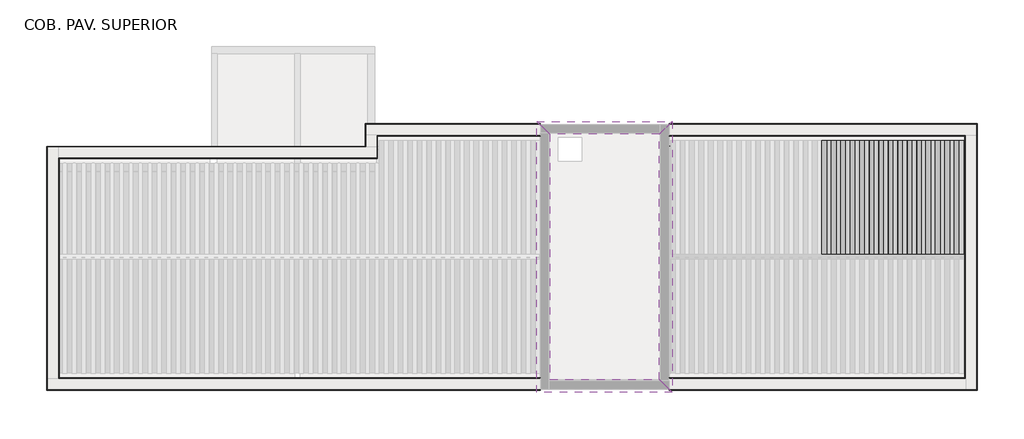
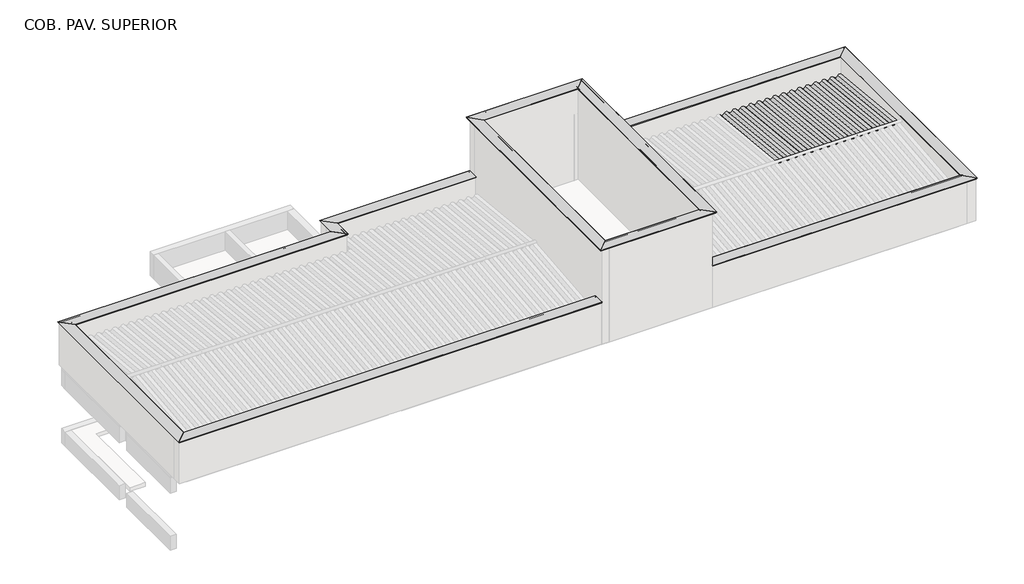
# One storey, part 7 of 7: 25 beams, 9 columns, 4 proxies.
"""IFC4 building model written with IfcOpenShell, lengths in millimetres."""

import ifcopenshell
import ifcopenshell.guid

model = None  # the IFC model being written
_history = None  # IfcOwnerHistory: only IFC2X3 demands one
_inside = {}  # id of a spatial element -> (the spatial element, [elements in it])
_under = {}  # id of a project, library or spatial element -> (it, [spatial elements below it])
_declared = {}  # id of a project -> (the project, [libraries it declares])
_typed = {}  # id of a type object -> (the type object, [elements of that type])
_made_of = {}  # id of a material, layer set ... -> (it, [elements and type objects made of it])


def new_model(schema):
    """Start an empty IFC model of exactly this schema.

    Asked for "IFC4X3", IfcOpenShell would pick the latest addendum, in which some entities
    have other attributes; the version numbers below select the first issue.
    IFC2X3 requires an IfcOwnerHistory on every rooted entity: one is made here for all.
    """
    global model, _history
    if schema == "IFC4X3":
        model = ifcopenshell.file(schema_version=(4, 3, 0, 0))
    else:
        model = ifcopenshell.file(schema=schema)
    _inside.clear()
    _under.clear()
    _declared.clear()
    _typed.clear()
    _made_of.clear()
    _history = None
    if model.schema == "IFC2X3":
        org = make("IfcOrganization", Name="unknown")
        user = make(
            "IfcPersonAndOrganization",
            ThePerson=make("IfcPerson", FamilyName="unknown"),
            TheOrganization=org,
        )
        app = make(
            "IfcApplication",
            ApplicationDeveloper=org,
            Version="unknown",
            ApplicationFullName="unknown",
            ApplicationIdentifier="unknown",
        )
        _history = make(
            "IfcOwnerHistory",
            OwningUser=user,
            OwningApplication=app,
            ChangeAction="ADDED",
            CreationDate=0,
        )
    return model


def make(cls, **values):
    """One entity of the class cls with the attributes given. An attribute that is None is left unset."""
    return model.create_entity(
        cls, **{name: value for name, value in values.items() if value is not None}
    )


def rooted(cls, **values):
    """An entity with a GlobalId (a new one), such as an element, a storey or a relation."""
    return make(cls, GlobalId=ifcopenshell.guid.new(), OwnerHistory=_history, **values)


def si_unit(unit_type, name, prefix=None):
    """IfcSIUnit, for example si_unit("LENGTHUNIT", "METRE", prefix="MILLI")."""
    return make("IfcSIUnit", UnitType=unit_type, Prefix=prefix, Name=name)


def assignment(units):
    """IfcUnitAssignment: the units of a project."""
    return None if units is None else make("IfcUnitAssignment", Units=units)


def point(xyz):
    """IfcCartesianPoint."""
    return None if xyz is None else make("IfcCartesianPoint", Coordinates=xyz)


def direction(xyz):
    """IfcDirection."""
    return None if xyz is None else make("IfcDirection", DirectionRatios=xyz)


def frame(location, z_axis=None, x_axis=None):
    """IfcAxis2Placement3D, a coordinate frame: its origin and axes. An axis left out is left unset."""
    return make(
        "IfcAxis2Placement3D",
        Location=point(location),
        Axis=direction(z_axis),
        RefDirection=direction(x_axis),
    )


def frame_2d(location, x_axis=None):
    """IfcAxis2Placement2D, a coordinate frame in the plane: its origin and x axis."""
    return make(
        "IfcAxis2Placement2D", Location=point(location), RefDirection=direction(x_axis)
    )


def origin():
    """The frame at (0, 0, 0) with its axes left unset."""
    return frame((0.0, 0.0, 0.0))


def place(relative_to, where):
    """IfcLocalPlacement: puts the frame where relative to a parent placement (None: the world)."""
    return make(
        "IfcLocalPlacement", PlacementRelTo=relative_to, RelativePlacement=where
    )


def context(
    kind, dimensions, precision=None, world=None, true_north=None, identifier=None
):
    """IfcGeometricRepresentationContext, for example the 3D "Model" context."""
    return make(
        "IfcGeometricRepresentationContext",
        ContextIdentifier=identifier,
        ContextType=kind,
        CoordinateSpaceDimension=dimensions,
        Precision=precision,
        WorldCoordinateSystem=world,
        TrueNorth=true_north,
    )


def project(units=None, contexts=None):
    """IfcProject with its units and contexts."""
    return rooted(
        "IfcProject",
        Name="project",
        RepresentationContexts=contexts,
        UnitsInContext=assignment(units),
    )


def spatial(cls, under=None, at=None, **own):
    """A site, building, storey or space (cls), placed at a placement, below another one or the project."""
    s = rooted(cls, ObjectPlacement=at, **own)
    if under is not None:
        _under.setdefault(under.id(), (under, []))[1].append(s)
    return s


def polyline(points):
    """IfcPolyline through the points."""
    return make("IfcPolyline", Points=[point(p) for p in points])


def circle_curve(where, radius):
    """IfcCircle in the frame where."""
    return make("IfcCircle", Position=where, Radius=radius)


def trimmed(basis, trim1, trim2, sense, master):
    """IfcTrimmedCurve: the piece of a basis curve between two trims."""
    return make(
        "IfcTrimmedCurve",
        BasisCurve=basis,
        Trim1=trim1,
        Trim2=trim2,
        SenseAgreement=sense,
        MasterRepresentation=master,
    )


def segment(curve, same_sense, transition):
    """IfcCompositeCurveSegment."""
    return make(
        "IfcCompositeCurveSegment",
        Transition=transition,
        SameSense=same_sense,
        ParentCurve=curve,
    )


def composite_curve(segments, self_intersect=None):
    """IfcCompositeCurve: segments joined end to end."""
    return make("IfcCompositeCurve", Segments=segments, SelfIntersect=self_intersect)


def outline(outer, holes=None, kind="AREA"):
    """IfcArbitraryClosedProfileDef: a profile drawn as a closed curve; with holes, ...WithVoids."""
    if holes is None:
        return make("IfcArbitraryClosedProfileDef", ProfileType=kind, OuterCurve=outer)
    return make(
        "IfcArbitraryProfileDefWithVoids",
        ProfileType=kind,
        OuterCurve=outer,
        InnerCurves=holes,
    )


def extrude(swept, where, along, depth):
    """IfcExtrudedAreaSolid: the profile swept, set in the frame where, extruded along a direction by depth."""
    return make(
        "IfcExtrudedAreaSolid",
        SweptArea=swept,
        Position=where,
        ExtrudedDirection=direction(along),
        Depth=depth,
    )


def faces_of(points, faces, orient=None, outer=None):
    """IfcFace entities. A face is a list of loops; a loop is a list of indices into points, from 0.

    orient and outer hold one flag for each loop. By default every Orientation is true, the
    first loop of a face is its IfcFaceOuterBound and the others are IfcFaceBound.
    """
    made = []
    for i, loops in enumerate(faces):
        bounds = []
        for j, loop in enumerate(loops):
            is_outer = j == 0 if outer is None else outer[i][j]
            bounds.append(
                make(
                    "IfcFaceOuterBound" if is_outer else "IfcFaceBound",
                    Bound=make("IfcPolyLoop", Polygon=[points[k] for k in loop]),
                    Orientation=True if orient is None else orient[i][j],
                )
            )
        made.append(make("IfcFace", Bounds=bounds))
    return made


def faceted_brep(points, faces, orient=None, outer=None, voids=None):
    """IfcFacetedBrep: a solid bounded by flat faces; with voids (closed shells), ...WithVoids."""
    shared = [point(p) for p in points]
    hull = make("IfcClosedShell", CfsFaces=faces_of(shared, faces, orient, outer))
    if voids is None:
        return make("IfcFacetedBrep", Outer=hull)
    return make(
        "IfcFacetedBrepWithVoids",
        Outer=hull,
        Voids=[
            make(cls, CfsFaces=faces_of(shared, fs, o, b)) for cls, fs, o, b in voids
        ],
    )


def shape(context_of_items, identifier, shape_type, items):
    """IfcShapeRepresentation: the items that make up one representation, for example the "Body"."""
    return make(
        "IfcShapeRepresentation",
        ContextOfItems=context_of_items,
        RepresentationIdentifier=identifier,
        RepresentationType=shape_type,
        Items=items,
    )


def source(mapping_origin, context_of_items, identifier, shape_type, items):
    """IfcRepresentationMap: a shape defined once, which mapped items show again and again."""
    return make(
        "IfcRepresentationMap",
        MappingOrigin=mapping_origin,
        MappedRepresentation=shape(context_of_items, identifier, shape_type, items),
    )


def transform(
    local_origin,
    x_axis=None,
    y_axis=None,
    z_axis=None,
    scale=None,
    scale2=None,
    scale3=None,
    uniform=True,
):
    """IfcCartesianTransformationOperator3D, or its non-uniform kind. x_axis, y_axis, z_axis: its Axis1, 2, 3."""
    if uniform:
        return make(
            "IfcCartesianTransformationOperator3D",
            Axis1=direction(x_axis),
            Axis2=direction(y_axis),
            LocalOrigin=point(local_origin),
            Scale=scale,
            Axis3=direction(z_axis),
        )
    return make(
        "IfcCartesianTransformationOperator3DnonUniform",
        Axis1=direction(x_axis),
        Axis2=direction(y_axis),
        LocalOrigin=point(local_origin),
        Scale=scale,
        Axis3=direction(z_axis),
        Scale2=scale2,
        Scale3=scale3,
    )


def mapped(mapping_source, mapping_target):
    """IfcMappedItem: shows the shape of a source again, moved by a transform."""
    return make(
        "IfcMappedItem", MappingSource=mapping_source, MappingTarget=mapping_target
    )


def made_of(thing, what):
    """Note that an element or type object is made of a material, layer set ...; save() writes the relation."""
    if what is not None:
        _made_of.setdefault(what.id(), (what, []))[1].append(thing)
    return thing


def element(
    cls,
    number,
    at=None,
    inside=None,
    cuts=None,
    type_object=None,
    material=None,
    context=None,
    identifier="Body",
    shape_type=None,
    held_by="IfcProductDefinitionShape",
    body=None,
    shapes=None,
    **own,
):
    """One element of the class cls, such as IfcWall. Its Tag is "e" and its number.

    at: its placement. inside: the storey or other place that contains it. cuts: it is an
    opening in that element (IfcRelVoidsElement). A single representation is given by context,
    identifier, shape_type and body (its items); several are given by shapes. held_by: the class
    of the entity that holds the representations. save() writes the other relations.
    """
    e = rooted(cls, Tag="e%d" % number, ObjectPlacement=at, **own)
    if body is not None:
        shapes = [shape(context, identifier, shape_type, body)]
    if shapes is not None:
        e.Representation = make(held_by, Representations=shapes)
    if inside is not None:
        _inside.setdefault(inside.id(), (inside, []))[1].append(e)
    if cuts is not None:
        rooted(
            "IfcRelVoidsElement", RelatingBuildingElement=cuts, RelatedOpeningElement=e
        )
    if type_object is not None:
        _typed.setdefault(type_object.id(), (type_object, []))[1].append(e)
    return made_of(e, material)


def aggregate(whole, parts):
    """IfcRelAggregates: a whole, such as a stair, and the parts it consists of."""
    return rooted("IfcRelAggregates", RelatingObject=whole, RelatedObjects=parts)


def save(model, path):
    """Write the relations noted so far, then the file.

    IfcRelAggregates (storeys below a building ...), IfcRelContainedInSpatialStructure (elements
    in a storey), IfcRelDefinesByType, IfcRelAssociatesMaterial and IfcRelDeclares: one each for
    every whole, place, type object, material and project.
    """
    for whole, parts in _under.values():
        aggregate(whole, parts)
    for where, things in _inside.values():
        rooted(
            "IfcRelContainedInSpatialStructure",
            RelatedElements=things,
            RelatingStructure=where,
        )
    for kind, things in _typed.values():
        rooted("IfcRelDefinesByType", RelatedObjects=things, RelatingType=kind)
    for what, things in _made_of.values():
        rooted("IfcRelAssociatesMaterial", RelatedObjects=things, RelatingMaterial=what)
    for by, libraries in _declared.values():
        rooted("IfcRelDeclares", RelatingContext=by, RelatedDefinitions=libraries)
    model.write(path)


def column_d505325c(model_context):
    return source(origin(), model_context, "Body", "SweptSolid", [
        extrude(outline(polyline([(30.0, 80.0), (30.0, -80.0), (-30.0, -80.0), (-30.0, 80.0), (30.0, 80.0)])), frame((0.0, 0.0, 6710.0), z_axis=(0.0, 0.0, 1.0), x_axis=(1.0, 0.0, 0.0)), (0.0, 0.0, 1.0), 750.0),
    ])


def column_4db371bd(model_context):
    return source(origin(), model_context, "Body", "SweptSolid", [
        extrude(outline(polyline([(30.0, 80.0), (30.0, -80.0), (-30.0, -80.0), (-30.0, 80.0), (30.0, 80.0)])), frame((0.0, 0.0, 6710.0), z_axis=(0.0, 0.0, 1.0), x_axis=(1.0, 0.0, 0.0)), (0.0, 0.0, 1.0), 660.0),
    ])


def column_d0cf395a(model_context):
    return source(origin(), model_context, "Body", "SweptSolid", [
        extrude(outline(polyline([(30.0, 80.0), (30.0, -80.0), (-30.0, -80.0), (-30.0, 80.0), (30.0, 80.0)])), frame((0.0, 0.0, 6710.0), z_axis=(0.0, 0.0, 1.0), x_axis=(1.0, 0.0, 0.0)), (0.0, 0.0, 1.0), 520.0),
    ])


model = new_model("IFC4")

# Units and contexts
model_context = context("Model", 3, world=origin())
ifc_project = project(units=[si_unit("LENGTHUNIT", "METRE", prefix="MILLI")], contexts=[model_context])

# Site, building, storey
site = spatial("IfcSite", under=ifc_project)
building = spatial("IfcBuilding", under=site)
storey = spatial("IfcBuildingStorey", under=building, Name="COB. PAV. SUPERIOR", Elevation=6650.0)

# Beams
placement = place(None, origin())
element("IfcBeam", 1, ObjectType="Madeira de lei : Berço 6x12cm", at=placement, inside=storey, context=model_context, shape_type="SweptSolid", body=[
    extrude(outline(polyline([(9090.718693, -7711.5607799), (9090.718693, -7831.5607799), (7090.718693, -7831.5607799), (7090.718693, -7711.5607799), (9090.718693, -7711.5607799)])), frame((0.0, 0.0, 6650.0), z_axis=(0.0, 0.0, 1.0), x_axis=(1.0, 0.0, 0.0)), (0.0, 0.0, 1.0), 60.0),
])
element("IfcBeam", 2, ObjectType="Madeira de lei : Berço 6x12cm", at=placement, inside=storey, context=model_context, shape_type="SweptSolid", body=[
    extrude(outline(polyline([(10730.718693, -7711.5607799), (10730.718693, -7831.5607799), (9090.718693, -7831.5607799), (9090.718693, -7711.5607799), (10730.718693, -7711.5607799)])), frame((0.0, 0.0, 6650.0), z_axis=(0.0, 0.0, 1.0), x_axis=(1.0, 0.0, 0.0)), (0.0, 0.0, 1.0), 60.0),
])
element("IfcBeam", 3, ObjectType="Madeira de lei : Berço 6x12cm", at=placement, inside=storey, context=model_context, shape_type="SweptSolid", body=[
    extrude(outline(polyline([(9089.7186924, -6319.8711004), (9089.7186924, -6439.8711004), (7089.7186936, -6439.8711004), (7089.7186936, -6319.8711004), (9089.7186924, -6319.8711004)])), frame((0.0, 0.0, 6650.0), z_axis=(0.0, 0.0, 1.0), x_axis=(1.0, 0.0, 0.0)), (0.0, 0.0, 1.0), 60.0),
])
element("IfcBeam", 4, ObjectType="Madeira de lei : Berço 6x12cm", at=placement, inside=storey, context=model_context, shape_type="SweptSolid", body=[
    extrude(outline(polyline([(10729.718693, -6319.8711004), (10729.718693, -6439.8711004), (9089.7186936, -6439.8711004), (9089.7186936, -6319.8711004), (10729.718693, -6319.8711004)])), frame((0.0, 0.0, 6650.0), z_axis=(0.0, 0.0, 1.0), x_axis=(1.0, 0.0, 0.0)), (0.0, 0.0, 1.0), 60.0),
])
element("IfcBeam", 5, ObjectType="Madeira de lei : Berço 6x12cm", at=placement, inside=storey, context=model_context, shape_type="SweptSolid", body=[
    extrude(outline(polyline([(5089.7186924, -4899.3026908), (5089.7186924, -5019.3026908), (3089.718693, -5019.3026908), (3089.718693, -4899.3026908), (5089.7186924, -4899.3026908)])), frame((0.0, 0.0, 6650.0), z_axis=(0.0, 0.0, 1.0), x_axis=(1.0, 0.0, 0.0)), (0.0, 0.0, 1.0), 60.0),
])
element("IfcBeam", 6, ObjectType="Madeira de lei : Berço 6x12cm", at=placement, inside=storey, context=model_context, shape_type="SweptSolid", body=[
    extrude(outline(polyline([(7089.7186924, -4899.3026908), (7089.7186924, -5019.3026908), (5089.7186936, -5019.3026908), (5089.7186936, -4899.3026908), (7089.7186924, -4899.3026908)])), frame((0.0, 0.0, 6650.0), z_axis=(0.0, 0.0, 1.0), x_axis=(1.0, 0.0, 0.0)), (0.0, 0.0, 1.0), 60.0),
])
element("IfcBeam", 7, ObjectType="Madeira de lei : Berço 6x12cm", at=placement, inside=storey, context=model_context, shape_type="SweptSolid", body=[
    extrude(outline(polyline([(9089.7186924, -4899.3026908), (9089.7186924, -5019.3026908), (7089.7186936, -5019.3026908), (7089.7186936, -4899.3026908), (9089.7186924, -4899.3026908)])), frame((0.0, 0.0, 6650.0), z_axis=(0.0, 0.0, 1.0), x_axis=(1.0, 0.0, 0.0)), (0.0, 0.0, 1.0), 60.0),
])
element("IfcBeam", 8, ObjectType="Madeira de lei : Berço 6x12cm", at=placement, inside=storey, context=model_context, shape_type="SweptSolid", body=[
    extrude(outline(polyline([(10729.718693, -4899.3026908), (10729.718693, -5019.3026908), (9089.7186936, -5019.3026908), (9089.7186936, -4899.3026908), (10729.718693, -4899.3026908)])), frame((0.0, 0.0, 6650.0), z_axis=(0.0, 0.0, 1.0), x_axis=(1.0, 0.0, 0.0)), (0.0, 0.0, 1.0), 60.0),
])
element("IfcBeam", 9, ObjectType="TQS - Viga retangular : 19.0 x 80.0", at=placement, inside=storey, context=model_context, shape_type="Brep", body=[
    faceted_brep([(10987.718693, -4565.5699847, 7250.0), (10797.718693, -4565.5699847, 7250.0), (10797.718693, -10953.5699847, 7250.0), (10987.718693, -10953.5699847, 7250.0), (10987.718693, -4565.5699847, 6450.0), (10987.718693, -10953.5699847, 6450.0), (10797.718693, -4565.5699847, 6450.0), (10797.718693, -10953.5699847, 6450.0), (10797.718693, -4565.5699847, 6650.0), (10797.718693, -10953.5699847, 6650.0)], [[[0, 1, 2, 3]], [[4, 0, 3, 5]], [[6, 4, 5, 7]], [[1, 8, 6, 7, 9, 2]], [[2, 9, 7, 5, 3]], [[1, 0, 4, 6, 8]]]),
])
element("IfcBeam", 10, ObjectType="TQS - Viga retangular : 19.0 x 80.0", at=placement, inside=storey, context=model_context, shape_type="Brep", body=[
    faceted_brep([(3049.718693, -4375.5518183, 7250.0), (3049.718693, -4565.5518183, 7250.0), (10637.718693, -4565.5067999, 7250.0), (10637.718693, -4375.5067999, 7250.0), (2749.718693, -4565.5535982, 7250.0), (-12.2807434, -4565.5699847, 7250.0), (-12.2807434, -4565.5699847, 6450.0), (10637.718693, -4565.5067999, 6450.0), (3049.718693, -4565.5518183, 6650.0), (2749.718693, -4565.5535982, 6650.0), (-12.2818706, -4375.5699847, 6450.0), (10637.718693, -4375.5067999, 6450.0), (-12.2818706, -4375.5699847, 7250.0), (2749.718693, -4375.5535982, 7250.0), (2749.7186931, -4375.5535982, 6650.0), (3049.718693, -4375.5518183, 6650.0)], [[[0, 1, 2, 3]], [[4, 5, 6, 7, 2, 1, 8, 9]], [[6, 10, 11, 7]], [[12, 13, 14, 15, 0, 3, 11, 10]], [[8, 15, 14, 9]], [[15, 8, 1, 0]], [[9, 14, 13, 4]], [[13, 12, 5, 4]], [[3, 2, 7, 11]], [[12, 10, 6, 5]]]),
])
element("IfcBeam", 11, ObjectType="Telha Ondulada : Fibrocimento", at=placement, inside=storey, context=model_context, shape_type="SweptSolid", body=[
    extrude(outline(composite_curve([segment(trimmed(circle_curve(frame_2d((-58.7002978, -53.2060539)), 66.7939461), [point((-29.3501489, 6.7939461))], [point((-29.3501489, -113.2060539))], False, "CARTESIAN"), True, "CONTINUOUS"), segment(polyline([(-29.3501489, -113.2060539), (-31.5472154, -108.7146289)]), True, "CONTINUOUS"), segment(trimmed(circle_curve(frame_2d((-58.7002978, -53.2060539)), 61.7939461), [point((-31.5472154, -108.7146289))], [point((-31.5472154, 2.3025211))], True, "CARTESIAN"), True, "CONTINUOUS"), segment(trimmed(circle_curve(frame_2d((0.0, 66.7939461)), 71.7939461), [point((-31.5472154, 2.3025211))], [point((-31.5472154, 131.2853711))], False, "CARTESIAN"), True, "CONTINUOUS"), segment(polyline([(-31.5472154, 131.2853711), (-29.3501489, 126.7939461)]), True, "CONTINUOUS"), segment(trimmed(circle_curve(frame_2d((0.0, 66.7939461)), 66.7939461), [point((-29.3501489, 126.7939461))], [point((-29.3501489, 6.7939461))], True, "CARTESIAN"), True, "CONTINUOUS")], self_intersect=False)), frame((7168.1156257, -4759.1621575, 7394.5315886), z_axis=(0.0, -0.9950371902099893, 0.09950371902099778), x_axis=(0.0, 0.09950371902099778, 0.9950371902099893)), (0.0, 0.0, 1.0), 3017.2387654),
])
element("IfcBeam", 12, ObjectType="Telha Ondulada : Fibrocimento", at=placement, inside=storey, context=model_context, shape_type="SweptSolid", body=[
    extrude(outline(composite_curve([segment(trimmed(circle_curve(frame_2d((-58.7002978, -53.2060539)), 66.7939461), [point((-29.3501489, 6.7939461))], [point((-29.3501489, -113.2060539))], False, "CARTESIAN"), True, "CONTINUOUS"), segment(polyline([(-29.3501489, -113.2060539), (-31.5472154, -108.7146289)]), True, "CONTINUOUS"), segment(trimmed(circle_curve(frame_2d((-58.7002978, -53.2060539)), 61.7939461), [point((-31.5472154, -108.7146289))], [point((-31.5472154, 2.3025211))], True, "CARTESIAN"), True, "CONTINUOUS"), segment(trimmed(circle_curve(frame_2d((0.0, 66.7939461)), 71.7939461), [point((-31.5472154, 2.3025211))], [point((-31.5472154, 131.2853711))], False, "CARTESIAN"), True, "CONTINUOUS"), segment(polyline([(-31.5472154, 131.2853711), (-29.3501489, 126.7939461)]), True, "CONTINUOUS"), segment(trimmed(circle_curve(frame_2d((0.0, 66.7939461)), 66.7939461), [point((-29.3501489, 126.7939461))], [point((-29.3501489, 6.7939461))], True, "CARTESIAN"), True, "CONTINUOUS")], self_intersect=False)), frame((7412.6156257, -4759.1621575, 7394.5315886), z_axis=(0.0, -0.9950371902099893, 0.09950371902099776), x_axis=(0.0, 0.09950371902099776, 0.9950371902099893)), (0.0, 0.0, 1.0), 3017.2387654),
])
element("IfcBeam", 13, ObjectType="Telha Ondulada : Fibrocimento", at=placement, inside=storey, context=model_context, shape_type="SweptSolid", body=[
    extrude(outline(composite_curve([segment(trimmed(circle_curve(frame_2d((-58.7002978, -53.2060539)), 66.7939461), [point((-29.3501489, 6.7939461))], [point((-29.3501489, -113.2060539))], False, "CARTESIAN"), True, "CONTINUOUS"), segment(polyline([(-29.3501489, -113.2060539), (-31.5472154, -108.7146289)]), True, "CONTINUOUS"), segment(trimmed(circle_curve(frame_2d((-58.7002978, -53.2060539)), 61.7939461), [point((-31.5472154, -108.7146289))], [point((-31.5472154, 2.3025211))], True, "CARTESIAN"), True, "CONTINUOUS"), segment(trimmed(circle_curve(frame_2d((0.0, 66.7939461)), 71.7939461), [point((-31.5472154, 2.3025211))], [point((-31.5472154, 131.2853711))], False, "CARTESIAN"), True, "CONTINUOUS"), segment(polyline([(-31.5472154, 131.2853711), (-29.3501489, 126.7939461)]), True, "CONTINUOUS"), segment(trimmed(circle_curve(frame_2d((0.0, 66.7939461)), 66.7939461), [point((-29.3501489, 126.7939461))], [point((-29.3501489, 6.7939461))], True, "CARTESIAN"), True, "CONTINUOUS")], self_intersect=False)), frame((7657.1156257, -4759.1621575, 7394.5315886), z_axis=(0.0, -0.9950371902099893, 0.09950371902099775), x_axis=(0.0, 0.09950371902099775, 0.9950371902099893)), (0.0, 0.0, 1.0), 3017.2387654),
])
element("IfcBeam", 14, ObjectType="Telha Ondulada : Fibrocimento", at=placement, inside=storey, context=model_context, shape_type="SweptSolid", body=[
    extrude(outline(composite_curve([segment(trimmed(circle_curve(frame_2d((-58.7002978, -53.2060539)), 66.7939461), [point((-29.3501489, 6.7939461))], [point((-29.3501489, -113.2060539))], False, "CARTESIAN"), True, "CONTINUOUS"), segment(polyline([(-29.3501489, -113.2060539), (-31.5472154, -108.7146289)]), True, "CONTINUOUS"), segment(trimmed(circle_curve(frame_2d((-58.7002978, -53.2060539)), 61.7939461), [point((-31.5472154, -108.7146289))], [point((-31.5472154, 2.3025211))], True, "CARTESIAN"), True, "CONTINUOUS"), segment(trimmed(circle_curve(frame_2d((0.0, 66.7939461)), 71.7939461), [point((-31.5472154, 2.3025211))], [point((-31.5472154, 131.2853711))], False, "CARTESIAN"), True, "CONTINUOUS"), segment(polyline([(-31.5472154, 131.2853711), (-29.3501489, 126.7939461)]), True, "CONTINUOUS"), segment(trimmed(circle_curve(frame_2d((0.0, 66.7939461)), 66.7939461), [point((-29.3501489, 126.7939461))], [point((-29.3501489, 6.7939461))], True, "CARTESIAN"), True, "CONTINUOUS")], self_intersect=False)), frame((7901.6156257, -4759.1621575, 7394.5315886), z_axis=(0.0, -0.9950371902099893, 0.09950371902099778), x_axis=(0.0, 0.09950371902099778, 0.9950371902099893)), (0.0, 0.0, 1.0), 3017.2387654),
])
element("IfcBeam", 15, ObjectType="Telha Ondulada : Fibrocimento", at=placement, inside=storey, context=model_context, shape_type="SweptSolid", body=[
    extrude(outline(composite_curve([segment(trimmed(circle_curve(frame_2d((-58.7002978, -53.2060539)), 66.7939461), [point((-29.3501489, 6.7939461))], [point((-29.3501489, -113.2060539))], False, "CARTESIAN"), True, "CONTINUOUS"), segment(polyline([(-29.3501489, -113.2060539), (-31.5472154, -108.7146289)]), True, "CONTINUOUS"), segment(trimmed(circle_curve(frame_2d((-58.7002978, -53.2060539)), 61.7939461), [point((-31.5472154, -108.7146289))], [point((-31.5472154, 2.3025211))], True, "CARTESIAN"), True, "CONTINUOUS"), segment(trimmed(circle_curve(frame_2d((0.0, 66.7939461)), 71.7939461), [point((-31.5472154, 2.3025211))], [point((-31.5472154, 131.2853711))], False, "CARTESIAN"), True, "CONTINUOUS"), segment(polyline([(-31.5472154, 131.2853711), (-29.3501489, 126.7939461)]), True, "CONTINUOUS"), segment(trimmed(circle_curve(frame_2d((0.0, 66.7939461)), 66.7939461), [point((-29.3501489, 126.7939461))], [point((-29.3501489, 6.7939461))], True, "CARTESIAN"), True, "CONTINUOUS")], self_intersect=False)), frame((8146.1156257, -4759.1621575, 7394.5315886), z_axis=(0.0, -0.9950371902099893, 0.09950371902099776), x_axis=(0.0, 0.09950371902099776, 0.9950371902099893)), (0.0, 0.0, 1.0), 3017.2387654),
])
element("IfcBeam", 16, ObjectType="Telha Ondulada : Fibrocimento", at=placement, inside=storey, context=model_context, shape_type="SweptSolid", body=[
    extrude(outline(composite_curve([segment(trimmed(circle_curve(frame_2d((-58.7002978, -53.2060539)), 66.7939461), [point((-29.3501489, 6.7939461))], [point((-29.3501489, -113.2060539))], False, "CARTESIAN"), True, "CONTINUOUS"), segment(polyline([(-29.3501489, -113.2060539), (-31.5472154, -108.7146289)]), True, "CONTINUOUS"), segment(trimmed(circle_curve(frame_2d((-58.7002978, -53.2060539)), 61.7939461), [point((-31.5472154, -108.7146289))], [point((-31.5472154, 2.3025211))], True, "CARTESIAN"), True, "CONTINUOUS"), segment(trimmed(circle_curve(frame_2d((0.0, 66.7939461)), 71.7939461), [point((-31.5472154, 2.3025211))], [point((-31.5472154, 131.2853711))], False, "CARTESIAN"), True, "CONTINUOUS"), segment(polyline([(-31.5472154, 131.2853711), (-29.3501489, 126.7939461)]), True, "CONTINUOUS"), segment(trimmed(circle_curve(frame_2d((0.0, 66.7939461)), 66.7939461), [point((-29.3501489, 126.7939461))], [point((-29.3501489, 6.7939461))], True, "CARTESIAN"), True, "CONTINUOUS")], self_intersect=False)), frame((8390.6156257, -4759.1621575, 7394.5315886), z_axis=(0.0, -0.9950371902099893, 0.09950371902099776), x_axis=(0.0, 0.09950371902099776, 0.9950371902099893)), (0.0, 0.0, 1.0), 3017.2387654),
])
element("IfcBeam", 17, ObjectType="Telha Ondulada : Fibrocimento", at=placement, inside=storey, context=model_context, shape_type="SweptSolid", body=[
    extrude(outline(composite_curve([segment(trimmed(circle_curve(frame_2d((-58.7002978, -53.2060539)), 66.7939461), [point((-29.3501489, 6.7939461))], [point((-29.3501489, -113.2060539))], False, "CARTESIAN"), True, "CONTINUOUS"), segment(polyline([(-29.3501489, -113.2060539), (-31.5472154, -108.7146289)]), True, "CONTINUOUS"), segment(trimmed(circle_curve(frame_2d((-58.7002978, -53.2060539)), 61.7939461), [point((-31.5472154, -108.7146289))], [point((-31.5472154, 2.3025211))], True, "CARTESIAN"), True, "CONTINUOUS"), segment(trimmed(circle_curve(frame_2d((0.0, 66.7939461)), 71.7939461), [point((-31.5472154, 2.3025211))], [point((-31.5472154, 131.2853711))], False, "CARTESIAN"), True, "CONTINUOUS"), segment(polyline([(-31.5472154, 131.2853711), (-29.3501489, 126.7939461)]), True, "CONTINUOUS"), segment(trimmed(circle_curve(frame_2d((0.0, 66.7939461)), 66.7939461), [point((-29.3501489, 126.7939461))], [point((-29.3501489, 6.7939461))], True, "CARTESIAN"), True, "CONTINUOUS")], self_intersect=False)), frame((8635.1156257, -4759.1621575, 7394.5315886), z_axis=(0.0, -0.9950371902099893, 0.09950371902099778), x_axis=(0.0, 0.09950371902099778, 0.9950371902099893)), (0.0, 0.0, 1.0), 3017.2387654),
])
element("IfcBeam", 18, ObjectType="Telha Ondulada : Fibrocimento", at=placement, inside=storey, context=model_context, shape_type="SweptSolid", body=[
    extrude(outline(composite_curve([segment(trimmed(circle_curve(frame_2d((-58.7002978, -53.2060539)), 66.7939461), [point((-29.3501489, 6.7939461))], [point((-29.3501489, -113.2060539))], False, "CARTESIAN"), True, "CONTINUOUS"), segment(polyline([(-29.3501489, -113.2060539), (-31.5472154, -108.7146289)]), True, "CONTINUOUS"), segment(trimmed(circle_curve(frame_2d((-58.7002978, -53.2060539)), 61.7939461), [point((-31.5472154, -108.7146289))], [point((-31.5472154, 2.3025211))], True, "CARTESIAN"), True, "CONTINUOUS"), segment(trimmed(circle_curve(frame_2d((0.0, 66.7939461)), 71.7939461), [point((-31.5472154, 2.3025211))], [point((-31.5472154, 131.2853711))], False, "CARTESIAN"), True, "CONTINUOUS"), segment(polyline([(-31.5472154, 131.2853711), (-29.3501489, 126.7939461)]), True, "CONTINUOUS"), segment(trimmed(circle_curve(frame_2d((0.0, 66.7939461)), 66.7939461), [point((-29.3501489, 126.7939461))], [point((-29.3501489, 6.7939461))], True, "CARTESIAN"), True, "CONTINUOUS")], self_intersect=False)), frame((8879.6156257, -4759.1621575, 7394.5315886), z_axis=(0.0, -0.9950371902099893, 0.09950371902099778), x_axis=(0.0, 0.09950371902099778, 0.9950371902099893)), (0.0, 0.0, 1.0), 3017.2387654),
])
element("IfcBeam", 19, ObjectType="Telha Ondulada : Fibrocimento", at=placement, inside=storey, context=model_context, shape_type="SweptSolid", body=[
    extrude(outline(composite_curve([segment(trimmed(circle_curve(frame_2d((-58.7002978, -53.2060539)), 66.7939461), [point((-29.3501489, 6.7939461))], [point((-29.3501489, -113.2060539))], False, "CARTESIAN"), True, "CONTINUOUS"), segment(polyline([(-29.3501489, -113.2060539), (-31.5472154, -108.7146289)]), True, "CONTINUOUS"), segment(trimmed(circle_curve(frame_2d((-58.7002978, -53.2060539)), 61.7939461), [point((-31.5472154, -108.7146289))], [point((-31.5472154, 2.3025211))], True, "CARTESIAN"), True, "CONTINUOUS"), segment(trimmed(circle_curve(frame_2d((0.0, 66.7939461)), 71.7939461), [point((-31.5472154, 2.3025211))], [point((-31.5472154, 131.2853711))], False, "CARTESIAN"), True, "CONTINUOUS"), segment(polyline([(-31.5472154, 131.2853711), (-29.3501489, 126.7939461)]), True, "CONTINUOUS"), segment(trimmed(circle_curve(frame_2d((0.0, 66.7939461)), 66.7939461), [point((-29.3501489, 126.7939461))], [point((-29.3501489, 6.7939461))], True, "CARTESIAN"), True, "CONTINUOUS")], self_intersect=False)), frame((9124.1156257, -4759.1621575, 7394.5315886), z_axis=(0.0, -0.9950371902099893, 0.09950371902099776), x_axis=(0.0, 0.09950371902099776, 0.9950371902099893)), (0.0, 0.0, 1.0), 3017.2387654),
])
element("IfcBeam", 20, ObjectType="Telha Ondulada : Fibrocimento", at=placement, inside=storey, context=model_context, shape_type="SweptSolid", body=[
    extrude(outline(composite_curve([segment(trimmed(circle_curve(frame_2d((-58.7002978, -53.2060539)), 66.7939461), [point((-29.3501489, 6.7939461))], [point((-29.3501489, -113.2060539))], False, "CARTESIAN"), True, "CONTINUOUS"), segment(polyline([(-29.3501489, -113.2060539), (-31.5472154, -108.7146289)]), True, "CONTINUOUS"), segment(trimmed(circle_curve(frame_2d((-58.7002978, -53.2060539)), 61.7939461), [point((-31.5472154, -108.7146289))], [point((-31.5472154, 2.3025211))], True, "CARTESIAN"), True, "CONTINUOUS"), segment(trimmed(circle_curve(frame_2d((0.0, 66.7939461)), 71.7939461), [point((-31.5472154, 2.3025211))], [point((-31.5472154, 131.2853711))], False, "CARTESIAN"), True, "CONTINUOUS"), segment(polyline([(-31.5472154, 131.2853711), (-29.3501489, 126.7939461)]), True, "CONTINUOUS"), segment(trimmed(circle_curve(frame_2d((0.0, 66.7939461)), 66.7939461), [point((-29.3501489, 126.7939461))], [point((-29.3501489, 6.7939461))], True, "CARTESIAN"), True, "CONTINUOUS")], self_intersect=False)), frame((9368.6156257, -4759.1621575, 7394.5315886), z_axis=(0.0, -0.9950371902099893, 0.09950371902099776), x_axis=(0.0, 0.09950371902099776, 0.9950371902099893)), (0.0, 0.0, 1.0), 3017.2387654),
])
element("IfcBeam", 21, ObjectType="Telha Ondulada : Fibrocimento", at=placement, inside=storey, context=model_context, shape_type="SweptSolid", body=[
    extrude(outline(composite_curve([segment(trimmed(circle_curve(frame_2d((-58.7002978, -53.2060539)), 66.7939461), [point((-29.3501489, 6.7939461))], [point((-29.3501489, -113.2060539))], False, "CARTESIAN"), True, "CONTINUOUS"), segment(polyline([(-29.3501489, -113.2060539), (-31.5472154, -108.7146289)]), True, "CONTINUOUS"), segment(trimmed(circle_curve(frame_2d((-58.7002978, -53.2060539)), 61.7939461), [point((-31.5472154, -108.7146289))], [point((-31.5472154, 2.3025211))], True, "CARTESIAN"), True, "CONTINUOUS"), segment(trimmed(circle_curve(frame_2d((0.0, 66.7939461)), 71.7939461), [point((-31.5472154, 2.3025211))], [point((-31.5472154, 131.2853711))], False, "CARTESIAN"), True, "CONTINUOUS"), segment(polyline([(-31.5472154, 131.2853711), (-29.3501489, 126.7939461)]), True, "CONTINUOUS"), segment(trimmed(circle_curve(frame_2d((0.0, 66.7939461)), 66.7939461), [point((-29.3501489, 126.7939461))], [point((-29.3501489, 6.7939461))], True, "CARTESIAN"), True, "CONTINUOUS")], self_intersect=False)), frame((9613.1156257, -4759.1621575, 7394.5315886), z_axis=(0.0, -0.9950371902099893, 0.09950371902099775), x_axis=(0.0, 0.09950371902099775, 0.9950371902099893)), (0.0, 0.0, 1.0), 3017.2387654),
])
element("IfcBeam", 22, ObjectType="Telha Ondulada : Fibrocimento", at=placement, inside=storey, context=model_context, shape_type="SweptSolid", body=[
    extrude(outline(composite_curve([segment(trimmed(circle_curve(frame_2d((-58.7002978, -53.2060539)), 66.7939461), [point((-29.3501489, 6.7939461))], [point((-29.3501489, -113.2060539))], False, "CARTESIAN"), True, "CONTINUOUS"), segment(polyline([(-29.3501489, -113.2060539), (-31.5472154, -108.7146289)]), True, "CONTINUOUS"), segment(trimmed(circle_curve(frame_2d((-58.7002978, -53.2060539)), 61.7939461), [point((-31.5472154, -108.7146289))], [point((-31.5472154, 2.3025211))], True, "CARTESIAN"), True, "CONTINUOUS"), segment(trimmed(circle_curve(frame_2d((0.0, 66.7939461)), 71.7939461), [point((-31.5472154, 2.3025211))], [point((-31.5472154, 131.2853711))], False, "CARTESIAN"), True, "CONTINUOUS"), segment(polyline([(-31.5472154, 131.2853711), (-29.3501489, 126.7939461)]), True, "CONTINUOUS"), segment(trimmed(circle_curve(frame_2d((0.0, 66.7939461)), 66.7939461), [point((-29.3501489, 126.7939461))], [point((-29.3501489, 6.7939461))], True, "CARTESIAN"), True, "CONTINUOUS")], self_intersect=False)), frame((9857.6156257, -4759.1621575, 7394.5315886), z_axis=(0.0, -0.9950371902099893, 0.09950371902099778), x_axis=(0.0, 0.09950371902099778, 0.9950371902099893)), (0.0, 0.0, 1.0), 3017.2387654),
])
element("IfcBeam", 23, ObjectType="Telha Ondulada : Fibrocimento", at=placement, inside=storey, context=model_context, shape_type="SweptSolid", body=[
    extrude(outline(composite_curve([segment(trimmed(circle_curve(frame_2d((-58.7002978, -53.2060539)), 66.7939461), [point((-29.3501489, 6.7939461))], [point((-29.3501489, -113.2060539))], False, "CARTESIAN"), True, "CONTINUOUS"), segment(polyline([(-29.3501489, -113.2060539), (-31.5472154, -108.7146289)]), True, "CONTINUOUS"), segment(trimmed(circle_curve(frame_2d((-58.7002978, -53.2060539)), 61.7939461), [point((-31.5472154, -108.7146289))], [point((-31.5472154, 2.3025211))], True, "CARTESIAN"), True, "CONTINUOUS"), segment(trimmed(circle_curve(frame_2d((0.0, 66.7939461)), 71.7939461), [point((-31.5472154, 2.3025211))], [point((-31.5472154, 131.2853711))], False, "CARTESIAN"), True, "CONTINUOUS"), segment(polyline([(-31.5472154, 131.2853711), (-29.3501489, 126.7939461)]), True, "CONTINUOUS"), segment(trimmed(circle_curve(frame_2d((0.0, 66.7939461)), 66.7939461), [point((-29.3501489, 126.7939461))], [point((-29.3501489, 6.7939461))], True, "CARTESIAN"), True, "CONTINUOUS")], self_intersect=False)), frame((10102.1156257, -4759.1621575, 7394.5315886), z_axis=(0.0, -0.9950371902099893, 0.09950371902099776), x_axis=(0.0, 0.09950371902099776, 0.9950371902099893)), (0.0, 0.0, 1.0), 3017.2387654),
])
element("IfcBeam", 24, ObjectType="Telha Ondulada : Fibrocimento", at=placement, inside=storey, context=model_context, shape_type="SweptSolid", body=[
    extrude(outline(composite_curve([segment(trimmed(circle_curve(frame_2d((-58.7002978, -53.2060539)), 66.7939461), [point((-29.3501489, 6.7939461))], [point((-29.3501489, -113.2060539))], False, "CARTESIAN"), True, "CONTINUOUS"), segment(polyline([(-29.3501489, -113.2060539), (-31.5472154, -108.7146289)]), True, "CONTINUOUS"), segment(trimmed(circle_curve(frame_2d((-58.7002978, -53.2060539)), 61.7939461), [point((-31.5472154, -108.7146289))], [point((-31.5472154, 2.3025211))], True, "CARTESIAN"), True, "CONTINUOUS"), segment(trimmed(circle_curve(frame_2d((0.0, 66.7939461)), 71.7939461), [point((-31.5472154, 2.3025211))], [point((-31.5472154, 131.2853711))], False, "CARTESIAN"), True, "CONTINUOUS"), segment(polyline([(-31.5472154, 131.2853711), (-29.3501489, 126.7939461)]), True, "CONTINUOUS"), segment(trimmed(circle_curve(frame_2d((0.0, 66.7939461)), 66.7939461), [point((-29.3501489, 126.7939461))], [point((-29.3501489, 6.7939461))], True, "CARTESIAN"), True, "CONTINUOUS")], self_intersect=False)), frame((10346.6156257, -4759.1621575, 7394.5315886), z_axis=(0.0, -0.9950371902099893, 0.09950371902099776), x_axis=(0.0, 0.09950371902099776, 0.9950371902099893)), (0.0, 0.0, 1.0), 3017.2387654),
])
element("IfcBeam", 25, ObjectType="Telha Ondulada : Fibrocimento", at=placement, inside=storey, context=model_context, shape_type="SweptSolid", body=[
    extrude(outline(composite_curve([segment(trimmed(circle_curve(frame_2d((-58.7002978, -53.2060539)), 66.7939461), [point((-29.3501489, 6.7939461))], [point((-29.3501489, -113.2060539))], False, "CARTESIAN"), True, "CONTINUOUS"), segment(polyline([(-29.3501489, -113.2060539), (-31.5472154, -108.7146289)]), True, "CONTINUOUS"), segment(trimmed(circle_curve(frame_2d((-58.7002978, -53.2060539)), 61.7939461), [point((-31.5472154, -108.7146289))], [point((-31.5472154, 2.3025211))], True, "CARTESIAN"), True, "CONTINUOUS"), segment(trimmed(circle_curve(frame_2d((0.0, 66.7939461)), 71.7939461), [point((-31.5472154, 2.3025211))], [point((-31.5472154, 131.2853711))], False, "CARTESIAN"), True, "CONTINUOUS"), segment(polyline([(-31.5472154, 131.2853711), (-29.3501489, 126.7939461)]), True, "CONTINUOUS"), segment(trimmed(circle_curve(frame_2d((0.0, 66.7939461)), 66.7939461), [point((-29.3501489, 126.7939461))], [point((-29.3501489, 6.7939461))], True, "CARTESIAN"), True, "CONTINUOUS")], self_intersect=False)), frame((10591.1156257, -4759.1621575, 7394.5315886), z_axis=(0.0, -0.9950371902099893, 0.09950371902099778), x_axis=(0.0, 0.09950371902099778, 0.9950371902099893)), (0.0, 0.0, 1.0), 3017.2387654),
])

# Proxies
element("IfcBuildingElementProxy", 26, Name=".CC_RUFO_PINGADEIRA_27 cm", ObjectType=".CC_RUFO_PINGADEIRA_27 cm", at=placement, inside=storey, context=model_context, shape_type="Brep", body=[
    faceted_brep([(-4754.5024445, -4334.3488472, 7826.6820963), (-4747.4313766, -4341.419915, 7833.7531641), (-4747.4313766, -4341.419915, 7836.5815912), (-4754.0054581, -4334.8458336, 7830.0075098), (-4769.952748, -4318.8985437, 7860.0), (-4443.6098659, -4645.2414257, 7860.0), (-4459.5571559, -4629.2941358, 7830.0075098), (-4466.1312373, -4622.7200544, 7836.5815912), (-4466.1312373, -4622.7200544, 7833.7531641), (-4459.0601695, -4629.7911222, 7826.6820963), (-4440.281307, -4648.5699847, 7862.0), (-4773.281307, -4315.5699847, 7862.0), (-243.281307, -4334.3488472, 7826.6820963), (-243.281307, -4315.5699847, 7862.0), (-243.281307, -4648.5699847, 7862.0), (-243.281307, -4629.7911222, 7826.6820963), (-243.281307, -4622.7200544, 7833.7531641), (-243.281307, -4622.7200544, 7836.5815912), (-243.281307, -4629.2941358, 7830.0075098), (-243.281307, -4645.2414257, 7860.0), (-243.281307, -4318.8985437, 7860.0), (-243.281307, -4334.8458336, 7830.0075098), (-243.281307, -4341.419915, 7836.5815912), (-243.281307, -4341.419915, 7833.7531641)], [[[0, 1, 2, 3, 4, 5, 6, 7, 8, 9, 10, 11]], [[12, 13, 14, 15, 16, 17, 18, 19, 20, 21, 22, 23]], [[1, 0, 12, 23]], [[2, 1, 23, 22]], [[3, 2, 22, 21]], [[4, 3, 21, 20]], [[5, 4, 20, 19]], [[6, 5, 19, 18]], [[7, 6, 18, 17]], [[8, 7, 17, 16]], [[9, 8, 16, 15]], [[10, 9, 15, 14]], [[11, 10, 14, 13]], [[0, 11, 13, 12]]]),
    faceted_brep([(-4754.5024445, -4923.3488472, 7826.6820963), (-4747.4313766, -4930.419915, 7833.7531641), (-4747.4313766, -4930.419915, 7836.5815912), (-4754.0054581, -4923.8458336, 7830.0075098), (-4769.952748, -4907.8985437, 7860.0), (-4443.6098659, -5234.2414257, 7860.0), (-4459.5571559, -5218.2941358, 7830.0075098), (-4466.1312373, -5211.7200544, 7836.5815912), (-4466.1312373, -5211.7200544, 7833.7531641), (-4459.0601695, -5218.7911222, 7826.6820963), (-4440.281307, -5237.5699847, 7862.0), (-4773.281307, -4904.5699847, 7862.0), (-4754.5024445, -4334.3488472, 7826.6820963), (-4773.281307, -4315.5699847, 7862.0), (-4440.281307, -4648.5699847, 7862.0), (-4459.0601695, -4629.7911222, 7826.6820963), (-4466.1312373, -4622.7200544, 7833.7531641), (-4466.1312373, -4622.7200544, 7836.5815912), (-4459.5571559, -4629.2941358, 7830.0075098), (-4443.6098659, -4645.2414257, 7860.0), (-4769.952748, -4318.8985437, 7860.0), (-4754.0054581, -4334.8458336, 7830.0075098), (-4747.4313766, -4341.419915, 7836.5815912), (-4747.4313766, -4341.419915, 7833.7531641)], [[[0, 1, 2, 3, 4, 5, 6, 7, 8, 9, 10, 11]], [[12, 13, 14, 15, 16, 17, 18, 19, 20, 21, 22, 23]], [[1, 0, 12, 23]], [[2, 1, 23, 22]], [[3, 2, 22, 21]], [[4, 3, 21, 20]], [[5, 4, 20, 19]], [[6, 5, 19, 18]], [[7, 6, 18, 17]], [[8, 7, 17, 16]], [[9, 8, 16, 15]], [[10, 9, 15, 14]], [[11, 10, 14, 13]], [[0, 11, 13, 12]]]),
    faceted_brep([(-12982.5024444, -4923.3488472, 7826.6820963), (-12975.4313766, -4930.419915, 7833.7531641), (-12975.4313766, -4930.419915, 7836.5815912), (-12982.0054581, -4923.8458336, 7830.0075098), (-12997.952748, -4907.8985437, 7860.0), (-12671.6098659, -5234.2414257, 7860.0), (-12687.5571558, -5218.2941358, 7830.0075098), (-12694.1312373, -5211.7200544, 7836.5815912), (-12694.1312373, -5211.7200544, 7833.7531641), (-12687.0601695, -5218.7911222, 7826.6820963), (-12668.2813069, -5237.5699847, 7862.0), (-13001.2813069, -4904.5699847, 7862.0), (-4754.5024445, -4923.3488472, 7826.6820963), (-4773.281307, -4904.5699847, 7862.0), (-4440.281307, -5237.5699847, 7862.0), (-4459.0601695, -5218.7911222, 7826.6820963), (-4466.1312373, -5211.7200544, 7833.7531641), (-4466.1312373, -5211.7200544, 7836.5815912), (-4459.5571559, -5218.2941358, 7830.0075098), (-4443.6098659, -5234.2414257, 7860.0), (-4769.952748, -4907.8985437, 7860.0), (-4754.0054581, -4923.8458336, 7830.0075098), (-4747.4313766, -4930.419915, 7836.5815912), (-4747.4313766, -4930.419915, 7833.7531641)], [[[0, 1, 2, 3, 4, 5, 6, 7, 8, 9, 10, 11]], [[12, 13, 14, 15, 16, 17, 18, 19, 20, 21, 22, 23]], [[1, 0, 12, 23]], [[2, 1, 23, 22]], [[3, 2, 22, 21]], [[4, 3, 21, 20]], [[5, 4, 20, 19]], [[6, 5, 19, 18]], [[7, 6, 18, 17]], [[8, 7, 17, 16]], [[9, 8, 16, 15]], [[10, 9, 15, 14]], [[11, 10, 14, 13]], [[0, 11, 13, 12]]]),
    faceted_brep([(-12982.5024444, -11206.7911222, 7826.6820963), (-12975.4313766, -11199.7200544, 7833.7531641), (-12975.4313766, -11199.7200544, 7836.5815912), (-12982.0054581, -11206.2941358, 7830.0075098), (-12997.952748, -11222.2414257, 7860.0), (-12671.6098659, -10895.8985437, 7860.0), (-12687.5571558, -10911.8458336, 7830.0075098), (-12694.1312373, -10918.419915, 7836.5815912), (-12694.1312373, -10918.419915, 7833.7531641), (-12687.0601695, -10911.3488472, 7826.6820963), (-12668.2813069, -10892.5699847, 7862.0), (-13001.2813069, -11225.5699847, 7862.0), (-12982.5024444, -4923.3488472, 7826.6820963), (-13001.2813069, -4904.5699847, 7862.0), (-12668.2813069, -5237.5699847, 7862.0), (-12687.0601695, -5218.7911222, 7826.6820963), (-12694.1312373, -5211.7200544, 7833.7531641), (-12694.1312373, -5211.7200544, 7836.5815912), (-12687.5571558, -5218.2941358, 7830.0075098), (-12671.6098659, -5234.2414257, 7860.0), (-12997.952748, -4907.8985437, 7860.0), (-12982.0054581, -4923.8458336, 7830.0075098), (-12975.4313766, -4930.419915, 7836.5815912), (-12975.4313766, -4930.419915, 7833.7531641)], [[[0, 1, 2, 3, 4, 5, 6, 7, 8, 9, 10, 11]], [[12, 13, 14, 15, 16, 17, 18, 19, 20, 21, 22, 23]], [[1, 0, 12, 23]], [[2, 1, 23, 22]], [[3, 2, 22, 21]], [[4, 3, 21, 20]], [[5, 4, 20, 19]], [[6, 5, 19, 18]], [[7, 6, 18, 17]], [[8, 7, 17, 16]], [[9, 8, 16, 15]], [[10, 9, 15, 14]], [[11, 10, 14, 13]], [[0, 11, 13, 12]]]),
    faceted_brep([(-243.281307, -11206.7911222, 7826.6820963), (-243.281307, -11199.7200544, 7833.7531641), (-243.281307, -11199.7200544, 7836.5815912), (-243.281307, -11206.2941358, 7830.0075098), (-243.281307, -11222.2414257, 7860.0), (-243.281307, -10895.8985437, 7860.0), (-243.281307, -10911.8458336, 7830.0075098), (-243.281307, -10918.419915, 7836.5815912), (-243.281307, -10918.419915, 7833.7531641), (-243.281307, -10911.3488472, 7826.6820963), (-243.281307, -10892.5699847, 7862.0), (-243.281307, -11225.5699847, 7862.0), (-12982.5024444, -11206.7911222, 7826.6820963), (-13001.2813069, -11225.5699847, 7862.0), (-12668.2813069, -10892.5699847, 7862.0), (-12687.0601695, -10911.3488472, 7826.6820963), (-12694.1312373, -10918.419915, 7833.7531641), (-12694.1312373, -10918.419915, 7836.5815912), (-12687.5571558, -10911.8458336, 7830.0075098), (-12671.6098659, -10895.8985437, 7860.0), (-12997.952748, -11222.2414257, 7860.0), (-12982.0054581, -11206.2941358, 7830.0075098), (-12975.4313766, -11199.7200544, 7836.5815912), (-12975.4313766, -11199.7200544, 7833.7531641)], [[[0, 1, 2, 3, 4, 5, 6, 7, 8, 9, 10, 11]], [[12, 13, 14, 15, 16, 17, 18, 19, 20, 21, 22, 23]], [[1, 0, 12, 23]], [[2, 1, 23, 22]], [[3, 2, 22, 21]], [[4, 3, 21, 20]], [[5, 4, 20, 19]], [[6, 5, 19, 18]], [[7, 6, 18, 17]], [[8, 7, 17, 16]], [[9, 8, 16, 15]], [[10, 9, 15, 14]], [[11, 10, 14, 13]], [[0, 11, 13, 12]]]),
    faceted_brep([(11042.9398305, -11206.7911222, 7826.6820963), (11035.8687627, -11199.7200544, 7833.7531641), (11035.8687627, -11199.7200544, 7836.5815912), (11042.4428441, -11206.2941358, 7830.0075098), (11058.3901341, -11222.2414257, 7860.0), (10732.047252, -10895.8985437, 7860.0), (10747.9945419, -10911.8458336, 7830.0075098), (10754.5686234, -10918.419915, 7836.5815912), (10754.5686234, -10918.419915, 7833.7531641), (10747.4975555, -10911.3488472, 7826.6820963), (10728.718693, -10892.5699847, 7862.0), (11061.718693, -11225.5699847, 7862.0), (3090.718693, -11206.7911222, 7826.6820963), (3090.718693, -11225.5699847, 7862.0), (3090.718693, -10892.5699847, 7862.0), (3090.718693, -10911.3488472, 7826.6820963), (3090.718693, -10918.419915, 7833.7531641), (3090.718693, -10918.419915, 7836.5815912), (3090.718693, -10911.8458336, 7830.0075098), (3090.718693, -10895.8985437, 7860.0), (3090.718693, -11222.2414257, 7860.0), (3090.718693, -11206.2941358, 7830.0075098), (3090.718693, -11199.7200544, 7836.5815912), (3090.718693, -11199.7200544, 7833.7531641)], [[[0, 1, 2, 3, 4, 5, 6, 7, 8, 9, 10, 11]], [[12, 13, 14, 15, 16, 17, 18, 19, 20, 21, 22, 23]], [[1, 0, 12, 23]], [[2, 1, 23, 22]], [[3, 2, 22, 21]], [[4, 3, 21, 20]], [[5, 4, 20, 19]], [[6, 5, 19, 18]], [[7, 6, 18, 17]], [[8, 7, 17, 16]], [[9, 8, 16, 15]], [[10, 9, 15, 14]], [[11, 10, 14, 13]], [[0, 11, 13, 12]]]),
    faceted_brep([(11042.9398305, -4334.3304376, 7826.6820963), (11035.8687627, -4341.4015054, 7833.7531641), (11035.8687627, -4341.4015054, 7836.5815912), (11042.4428441, -4334.827424, 7830.0075098), (11058.3901341, -4318.8801341, 7860.0), (10732.047252, -4645.2230161, 7860.0), (10747.9945419, -4629.2757262, 7830.0075098), (10754.5686234, -4622.7016448, 7836.5815912), (10754.5686234, -4622.7016448, 7833.7531641), (10747.4975555, -4629.7727126, 7826.6820963), (10728.718693, -4648.5515751, 7862.0), (11061.718693, -4315.5515751, 7862.0), (11042.9398305, -11206.7911222, 7826.6820963), (11061.718693, -11225.5699847, 7862.0), (10728.718693, -10892.5699847, 7862.0), (10747.4975555, -10911.3488472, 7826.6820963), (10754.5686234, -10918.419915, 7833.7531641), (10754.5686234, -10918.419915, 7836.5815912), (10747.9945419, -10911.8458336, 7830.0075098), (10732.047252, -10895.8985437, 7860.0), (11058.3901341, -11222.2414257, 7860.0), (11042.4428441, -11206.2941358, 7830.0075098), (11035.8687627, -11199.7200544, 7836.5815912), (11035.8687627, -11199.7200544, 7833.7531641)], [[[0, 1, 2, 3, 4, 5, 6, 7, 8, 9, 10, 11]], [[12, 13, 14, 15, 16, 17, 18, 19, 20, 21, 22, 23]], [[1, 0, 12, 23]], [[2, 1, 23, 22]], [[3, 2, 22, 21]], [[4, 3, 21, 20]], [[5, 4, 20, 19]], [[6, 5, 19, 18]], [[7, 6, 18, 17]], [[8, 7, 17, 16]], [[9, 8, 16, 15]], [[10, 9, 15, 14]], [[11, 10, 14, 13]], [[0, 11, 13, 12]]]),
    faceted_brep([(3090.718693, -4334.3304376, 7826.6820963), (3090.718693, -4341.4015054, 7833.7531641), (3090.718693, -4341.4015054, 7836.5815912), (3090.718693, -4334.827424, 7830.0075098), (3090.718693, -4318.8801341, 7860.0), (3090.718693, -4645.2230161, 7860.0), (3090.718693, -4629.2757262, 7830.0075098), (3090.718693, -4622.7016448, 7836.5815912), (3090.718693, -4622.7016448, 7833.7531641), (3090.718693, -4629.7727126, 7826.6820963), (3090.718693, -4648.5515751, 7862.0), (3090.718693, -4315.5515751, 7862.0), (11042.9398305, -4334.3304376, 7826.6820963), (11061.718693, -4315.5515751, 7862.0), (10728.718693, -4648.5515751, 7862.0), (10747.4975555, -4629.7727126, 7826.6820963), (10754.5686234, -4622.7016448, 7833.7531641), (10754.5686234, -4622.7016448, 7836.5815912), (10747.9945419, -4629.2757262, 7830.0075098), (10732.047252, -4645.2230161, 7860.0), (11058.3901341, -4318.8801341, 7860.0), (11042.4428441, -4334.827424, 7830.0075098), (11035.8687627, -4341.4015054, 7836.5815912), (11035.8687627, -4341.4015054, 7833.7531641)], [[[0, 1, 2, 3, 4, 5, 6, 7, 8, 9, 10, 11]], [[12, 13, 14, 15, 16, 17, 18, 19, 20, 21, 22, 23]], [[1, 0, 12, 23]], [[2, 1, 23, 22]], [[3, 2, 22, 21]], [[4, 3, 21, 20]], [[5, 4, 20, 19]], [[6, 5, 19, 18]], [[7, 6, 18, 17]], [[8, 7, 17, 16]], [[9, 8, 16, 15]], [[10, 9, 15, 14]], [[11, 10, 14, 13]], [[0, 11, 13, 12]]]),
])
element("IfcBuildingElementProxy", 27, Name=".CC_RUFO_PINGADEIRA_27 cm", ObjectType=".CC_RUFO_PINGADEIRA_27 cm", at=placement, inside=storey, context=model_context, shape_type="Brep", body=[
    faceted_brep([(2857.4975555, -10962.3488472, 9526.6820963), (2838.718693, -10943.5699847, 9562.0), (3171.718693, -11276.5699847, 9562.0), (3152.9398305, -11257.7911222, 9526.6820963), (3145.8687627, -11250.7200544, 9533.7531641), (3145.8687627, -11250.7200544, 9536.5815912), (3152.4428441, -11257.2941358, 9530.0075098), (3168.3901341, -11273.2414257, 9560.0), (2842.047252, -10946.8985437, 9560.0), (2857.9945419, -10962.8458336, 9530.0075098), (2864.5686234, -10969.419915, 9536.5815912), (2864.5686234, -10969.419915, 9533.7531641), (-10.0601695, -10962.3488472, 9526.6820963), (-17.1312373, -10969.419915, 9533.7531641), (-17.1312373, -10969.419915, 9536.5815912), (-10.5571559, -10962.8458336, 9530.0075098), (5.3901341, -10946.8985437, 9560.0), (-320.952748, -11273.2414257, 9560.0), (-305.0054581, -11257.2941358, 9530.0075098), (-298.4313766, -11250.7200544, 9536.5815912), (-298.4313766, -11250.7200544, 9533.7531641), (-305.5024445, -11257.7911222, 9526.6820963), (-324.281307, -11276.5699847, 9562.0), (8.718693, -10943.5699847, 9562.0)], [[[0, 1, 2, 3, 4, 5, 6, 7, 8, 9, 10, 11]], [[12, 13, 14, 15, 16, 17, 18, 19, 20, 21, 22, 23]], [[1, 0, 12, 23]], [[2, 1, 23, 22]], [[3, 2, 22, 21]], [[4, 3, 21, 20]], [[5, 4, 20, 19]], [[6, 5, 19, 18]], [[7, 6, 18, 17]], [[8, 7, 17, 16]], [[9, 8, 16, 15]], [[10, 9, 15, 14]], [[11, 10, 14, 13]], [[0, 11, 13, 12]]]),
    faceted_brep([(-10.0601695, -10962.3488472, 9526.6820963), (8.718693, -10943.5699847, 9562.0), (-324.281307, -11276.5699847, 9562.0), (-305.5024445, -11257.7911222, 9526.6820963), (-298.4313766, -11250.7200544, 9533.7531641), (-298.4313766, -11250.7200544, 9536.5815912), (-305.0054581, -11257.2941358, 9530.0075098), (-320.952748, -11273.2414257, 9560.0), (5.3901341, -10946.8985437, 9560.0), (-10.5571559, -10962.8458336, 9530.0075098), (-17.1312373, -10969.419915, 9536.5815912), (-17.1312373, -10969.419915, 9533.7531641), (-10.0601695, -4578.7911222, 9526.6820963), (-17.1312373, -4571.7200544, 9533.7531641), (-17.1312373, -4571.7200544, 9536.5815912), (-10.5571559, -4578.2941358, 9530.0075098), (5.3901341, -4594.2414257, 9560.0), (-320.952748, -4267.8985437, 9560.0), (-305.0054581, -4283.8458336, 9530.0075098), (-298.4313766, -4290.419915, 9536.5815912), (-298.4313766, -4290.419915, 9533.7531641), (-305.5024445, -4283.3488472, 9526.6820963), (-324.281307, -4264.5699847, 9562.0), (8.718693, -4597.5699847, 9562.0)], [[[0, 1, 2, 3, 4, 5, 6, 7, 8, 9, 10, 11]], [[12, 13, 14, 15, 16, 17, 18, 19, 20, 21, 22, 23]], [[1, 0, 12, 23]], [[2, 1, 23, 22]], [[3, 2, 22, 21]], [[4, 3, 21, 20]], [[5, 4, 20, 19]], [[6, 5, 19, 18]], [[7, 6, 18, 17]], [[8, 7, 17, 16]], [[9, 8, 16, 15]], [[10, 9, 15, 14]], [[11, 10, 14, 13]], [[0, 11, 13, 12]]]),
])
element("IfcBuildingElementProxy", 28, Name=".CC_RUFO_PINGADEIRA_27 cm", ObjectType=".CC_RUFO_PINGADEIRA_27 cm", at=placement, inside=storey, context=model_context, shape_type="Brep", body=[
    faceted_brep([(-10.0601695, -4578.7911222, 9526.6820963), (8.718693, -4597.5699847, 9562.0), (-324.281307, -4264.5699847, 9562.0), (-305.5024445, -4283.3488472, 9526.6820963), (-298.4313766, -4290.419915, 9533.7531641), (-298.4313766, -4290.419915, 9536.5815912), (-305.0054581, -4283.8458336, 9530.0075098), (-320.952748, -4267.8985437, 9560.0), (5.3901341, -4594.2414257, 9560.0), (-10.5571559, -4578.2941358, 9530.0075098), (-17.1312373, -4571.7200544, 9536.5815912), (-17.1312373, -4571.7200544, 9533.7531641), (2857.4975555, -4578.7911222, 9526.6820963), (2864.5686234, -4571.7200544, 9533.7531641), (2864.5686234, -4571.7200544, 9536.5815912), (2857.9945419, -4578.2941358, 9530.0075098), (2842.047252, -4594.2414257, 9560.0), (3168.3901341, -4267.8985437, 9560.0), (3152.4428441, -4283.8458336, 9530.0075098), (3145.8687627, -4290.419915, 9536.5815912), (3145.8687627, -4290.419915, 9533.7531641), (3152.9398305, -4283.3488472, 9526.6820963), (3171.718693, -4264.5699847, 9562.0), (2838.718693, -4597.5699847, 9562.0)], [[[0, 1, 2, 3, 4, 5, 6, 7, 8, 9, 10, 11]], [[12, 13, 14, 15, 16, 17, 18, 19, 20, 21, 22, 23]], [[1, 0, 12, 23]], [[2, 1, 23, 22]], [[3, 2, 22, 21]], [[4, 3, 21, 20]], [[5, 4, 20, 19]], [[6, 5, 19, 18]], [[7, 6, 18, 17]], [[8, 7, 17, 16]], [[9, 8, 16, 15]], [[10, 9, 15, 14]], [[11, 10, 14, 13]], [[0, 11, 13, 12]]]),
])
element("IfcBuildingElementProxy", 29, Name=".CC_RUFO_PINGADEIRA_27 cm", ObjectType=".CC_RUFO_PINGADEIRA_27 cm", at=placement, inside=storey, context=model_context, shape_type="Brep", body=[
    faceted_brep([(2857.4975555, -4578.7911222, 9526.6820963), (2838.718693, -4597.5699847, 9562.0), (3171.718693, -4264.5699847, 9562.0), (3152.9398305, -4283.3488472, 9526.6820963), (3145.8687627, -4290.419915, 9533.7531641), (3145.8687627, -4290.419915, 9536.5815912), (3152.4428441, -4283.8458336, 9530.0075098), (3168.3901341, -4267.8985437, 9560.0), (2842.047252, -4594.2414257, 9560.0), (2857.9945419, -4578.2941358, 9530.0075098), (2864.5686234, -4571.7200544, 9536.5815912), (2864.5686234, -4571.7200544, 9533.7531641), (2857.4975555, -10962.3488472, 9526.6820963), (2864.5686234, -10969.419915, 9533.7531641), (2864.5686234, -10969.419915, 9536.5815912), (2857.9945419, -10962.8458336, 9530.0075098), (2842.047252, -10946.8985437, 9560.0), (3168.3901341, -11273.2414257, 9560.0), (3152.4428441, -11257.2941358, 9530.0075098), (3145.8687627, -11250.7200544, 9536.5815912), (3145.8687627, -11250.7200544, 9533.7531641), (3152.9398305, -11257.7911222, 9526.6820963), (3171.718693, -11276.5699847, 9562.0), (2838.718693, -10943.5699847, 9562.0)], [[[0, 1, 2, 3, 4, 5, 6, 7, 8, 9, 10, 11]], [[12, 13, 14, 15, 16, 17, 18, 19, 20, 21, 22, 23]], [[1, 0, 12, 23]], [[2, 1, 23, 22]], [[3, 2, 22, 21]], [[4, 3, 21, 20]], [[5, 4, 20, 19]], [[6, 5, 19, 18]], [[7, 6, 18, 17]], [[8, 7, 17, 16]], [[9, 8, 16, 15]], [[10, 9, 15, 14]], [[11, 10, 14, 13]], [[0, 11, 13, 12]]]),
])

# Columns
column_shape = column_d505325c(model_context)
element("IfcColumn", 30, ObjectType="Madeira de lei-Coluna : Pontalete 6X16cm", at=placement, inside=storey, context=model_context, shape_type="MappedRepresentation", body=[
    mapped(column_shape, transform((8090.718693, -7771.5607799, 0.0), x_axis=(0.0, 1.0, 0.0), y_axis=(-1.0, 0.0, 0.0), z_axis=(0.0, 0.0, 1.0))),
])
element("IfcColumn", 31, ObjectType="Madeira de lei-Coluna : Pontalete 6X16cm", at=placement, inside=storey, context=model_context, shape_type="MappedRepresentation", body=[
    mapped(column_shape, transform((10090.718693, -7771.5607799, 0.0), x_axis=(0.0, 1.0, 0.0), y_axis=(-1.0, 0.0, 0.0), z_axis=(0.0, 0.0, 1.0))),
])
column_2_shape = column_4db371bd(model_context)
element("IfcColumn", 32, ObjectType="Madeira de lei-Coluna : Pontalete 6X16cm", at=placement, inside=storey, context=model_context, shape_type="MappedRepresentation", body=[
    mapped(column_2_shape, transform((6089.718693, -6379.8711004, 0.0), x_axis=(0.0, 1.0, 0.0), y_axis=(-1.0, 0.0, 0.0), z_axis=(0.0, 0.0, 1.0))),
])
element("IfcColumn", 33, ObjectType="Madeira de lei-Coluna : Pontalete 6X16cm", at=placement, inside=storey, context=model_context, shape_type="MappedRepresentation", body=[
    mapped(column_2_shape, transform((8089.718693, -6379.8711004, 0.0), x_axis=(0.0, 1.0, 0.0), y_axis=(-1.0, 0.0, 0.0), z_axis=(0.0, 0.0, 1.0))),
])
element("IfcColumn", 34, ObjectType="Madeira de lei-Coluna : Pontalete 6X16cm", at=placement, inside=storey, context=model_context, shape_type="MappedRepresentation", body=[
    mapped(column_2_shape, transform((10089.718693, -6379.8711004, 0.0), x_axis=(0.0, 1.0, 0.0), y_axis=(-1.0, 0.0, 0.0), z_axis=(0.0, 0.0, 1.0))),
])
column_3_shape = column_d0cf395a(model_context)
element("IfcColumn", 35, ObjectType="Madeira de lei-Coluna : Pontalete 6X16cm", at=placement, inside=storey, context=model_context, shape_type="MappedRepresentation", body=[
    mapped(column_3_shape, transform((4089.718693, -4959.3026908, 0.0), x_axis=(0.0, 1.0, 0.0), y_axis=(-1.0, 0.0, 0.0), z_axis=(0.0, 0.0, 1.0))),
])
element("IfcColumn", 36, ObjectType="Madeira de lei-Coluna : Pontalete 6X16cm", at=placement, inside=storey, context=model_context, shape_type="MappedRepresentation", body=[
    mapped(column_3_shape, transform((6089.718693, -4959.3026908, 0.0), x_axis=(0.0, 1.0, 0.0), y_axis=(-1.0, 0.0, 0.0), z_axis=(0.0, 0.0, 1.0))),
])
element("IfcColumn", 37, ObjectType="Madeira de lei-Coluna : Pontalete 6X16cm", at=placement, inside=storey, context=model_context, shape_type="MappedRepresentation", body=[
    mapped(column_3_shape, transform((8089.718693, -4959.3026908, 0.0), x_axis=(0.0, 1.0, 0.0), y_axis=(-1.0, 0.0, 0.0), z_axis=(0.0, 0.0, 1.0))),
])
element("IfcColumn", 38, ObjectType="Madeira de lei-Coluna : Pontalete 6X16cm", at=placement, inside=storey, context=model_context, shape_type="MappedRepresentation", body=[
    mapped(column_3_shape, transform((10089.718693, -4959.3026908, 0.0), x_axis=(0.0, 1.0, 0.0), y_axis=(-1.0, 0.0, 0.0), z_axis=(0.0, 0.0, 1.0))),
])

save(model, "model.ifc")
